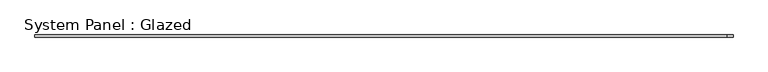
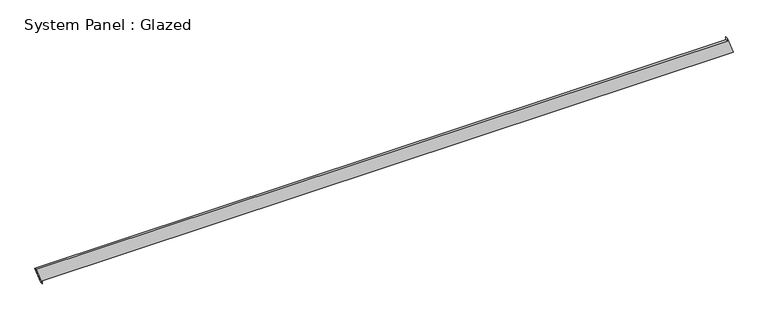
"""IFC4 building model written with IfcOpenShell, lengths in millimetres: plate geometry, System Panel : Glazed."""

from ifc_helpers import new_model, si_unit, frame, origin, place, context, project, spatial, polyline, outline, extrude, source, transform, mapped, element, save


def system_panel_glazed_9aac2072(model_context):
    return source(origin(), model_context, "Body", "SweptSolid", [
        extrude(outline(polyline([(0.0, -3959.0393549), (35.3553391, -3959.0393549), (35.3553391, 4028.0553276), (234.5588529, 3958.9170456), (199.2035139, 3958.9168202), (199.254446, -4028.0553276), (0.0, -3959.0393549)])), frame((0.0, -49.5, 0.0), z_axis=(0.0, 1.0, 0.0), x_axis=(0.0, 0.0, 1.0)), (0.0, 0.0, 1.0), 25.0),
    ])


if __name__ == "__main__":
    model = new_model("IFC4")
    model_context = context("Model", 3, world=origin())
    ifc_project = project(units=[si_unit("LENGTHUNIT", "METRE", prefix="MILLI")], contexts=[model_context])
    site = spatial("IfcSite", under=ifc_project)
    building = spatial("IfcBuilding", under=site)
    placement = place(None, origin())
    system_panel_glazed_shape = system_panel_glazed_9aac2072(model_context)
    element("IfcPlate", 1, ObjectType="System Panel : Glazed", at=placement, inside=building, context=model_context, shape_type="MappedRepresentation", body=[
        mapped(system_panel_glazed_shape, transform((0.0, 0.0, 0.0), x_axis=(1.0, 0.0, 0.0), y_axis=(0.0, 1.0, 0.0), z_axis=(0.0, 0.0, 1.0))),
    ])
    save(model, "model.ifc")

# Revit data of these elements
# Element 1 (IfcPlate, "System Panel : Glazed")
#   Materials on its faces: "Glass"
# Materials
#   "Glass": class "Glass", colour RGB 218 227 224, transparency 0.85, Description = "Soda Lime Glass", Cost = 0
